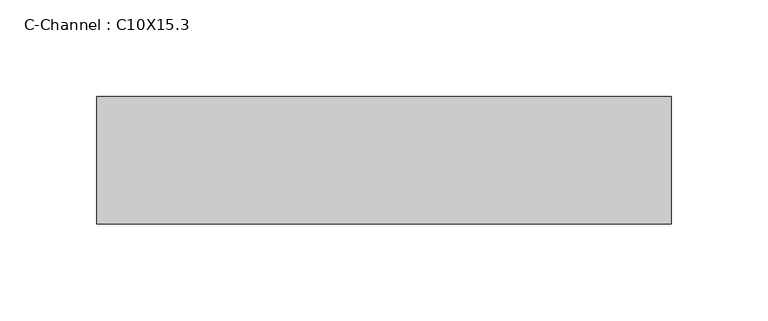
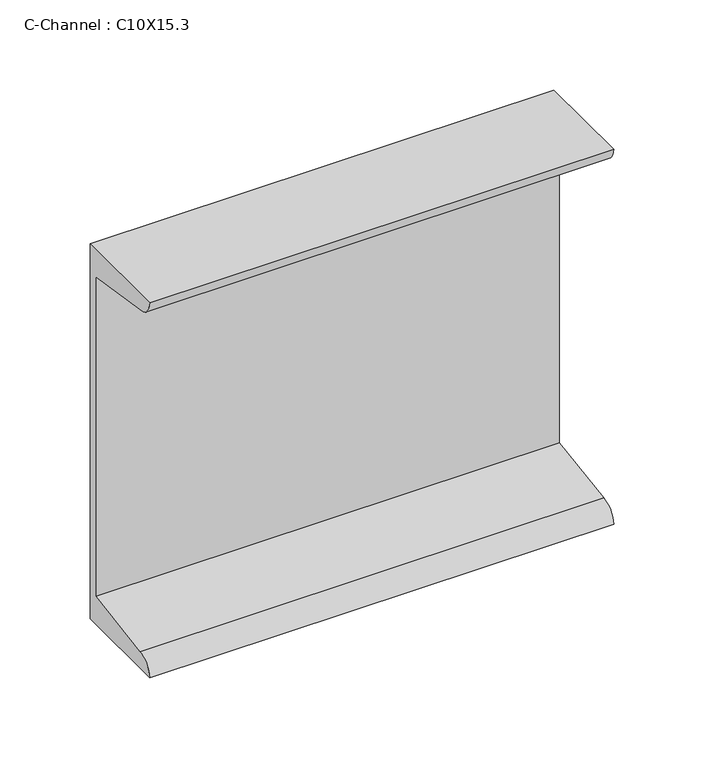
"""IFC4 building model written with IfcOpenShell, lengths in millimetres: beam geometry, C-Channel : C10X15.3."""

from ifc_helpers import new_model, si_unit, point, frame, frame_2d, origin, place, context, project, spatial, polyline, circle_curve, trimmed, segment, composite_curve, outline, extrude, source, transform, mapped, element, save


def c_channel_c10x15_3_3b12c983(model_context):
    return source(origin(), model_context, "Body", "SweptSolid", [
        extrude(outline(composite_curve([segment(polyline([(16.1036, 127.0), (16.1036, -127.0), (-49.9364, -127.0)]), True, "CONTINUOUS"), segment(trimmed(circle_curve(frame_2d((-38.862, -127.0)), 11.0744), [point((-49.9364, -127.0))], [point((-38.862, -115.9256))], False, "CARTESIAN"), True, "CONTINUOUS"), segment(polyline([(-38.862, -115.9256), (10.0076, -108.1854158), (10.0076, 108.1854158), (-38.862, 115.9256)]), True, "CONTINUOUS"), segment(trimmed(circle_curve(frame_2d((-38.862, 127.0)), 11.0744), [point((-38.862, 115.9256))], [point((-49.9364, 127.0))], False, "CARTESIAN"), True, "CONTINUOUS"), segment(polyline([(-49.9364, 127.0), (16.1036, 127.0)]), True, "CONTINUOUS")], self_intersect=False)), frame((-93.98, 0.0, 0.0), z_axis=(1.0, 0.0, 0.0), x_axis=(0.0, 1.0, 0.0)), (0.0, 0.0, 1.0), 297.18),
    ])


if __name__ == "__main__":
    model = new_model("IFC4")
    model_context = context("Model", 3, world=origin())
    ifc_project = project(units=[si_unit("LENGTHUNIT", "METRE", prefix="MILLI")], contexts=[model_context])
    site = spatial("IfcSite", under=ifc_project)
    building = spatial("IfcBuilding", under=site)
    placement = place(None, origin())
    c_channel_c10x15_3_shape = c_channel_c10x15_3_3b12c983(model_context)
    element("IfcBeam", 1, ObjectType="C-Channel : C10X15.3", at=placement, inside=building, context=model_context, shape_type="MappedRepresentation", body=[
        mapped(c_channel_c10x15_3_shape, transform((0.0, 0.0, 0.0), x_axis=(1.0, 0.0, 0.0), y_axis=(0.0, 1.0, 0.0), z_axis=(0.0, 0.0, 1.0))),
    ])
    save(model, "model.ifc")

# Revit data of these elements
# Type "C-Channel : C10X15.3"
#   Assembly Code = "B10"
#   W = 15.3
#   Length [instance default] = 5' - 0"
#   bf = 0' - 2.6"
#   d = 0' - 10"
#   tf = 0' - 0.436"
#   tw = 0' - 0.24"
#   x = 0' - 0.634"
#   A = 0.0311111 SF
#   Structural Material [instance default] = Steel ASTM A36
# Element 1 (IfcBeam, "C-Channel : C10X15.3")
#   Structural Material = Steel ASTM A992
#   Materials on its faces: "Steel ASTM A992"
# Materials
#   "Steel ASTM A36": class "Metal", colour RGB 199 199 199, transparency 0, Description = "Structural steel, ASTM A36 Grade B, mill finish", Cost = 0
#   "Steel ASTM A992": class "Metal", colour RGB 199 199 199, transparency 0, Description = "Structural steel 50ksi", Cost = 0
